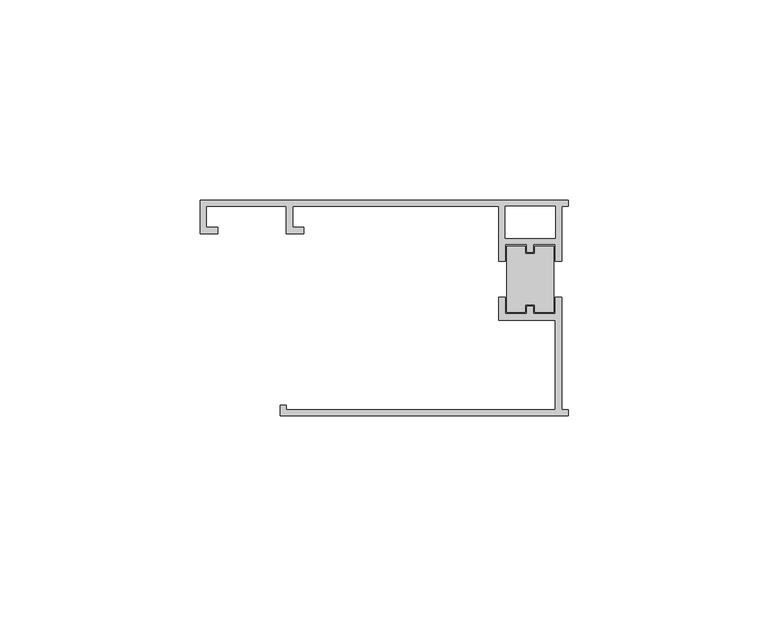
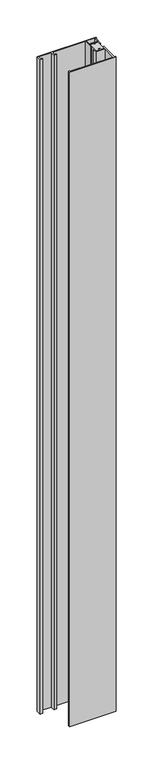
"""IFC4 building model written with IfcOpenShell, lengths in millimetres: proxy geometry, Generic Models 2:Generic Models 2:310765:Generic Models 2:310765 : Generic Models 2:Generic Models 2:310765:59 : Generic Models 2:Generic Models 2:310765:Generic Models 2:310765 : Generic Models 2:Generic Models 2:310765:300385."""

from ifc_helpers import new_model, si_unit, frame, origin, place, context, project, spatial, polyline, outline, extrude, source, transform, mapped, element, save


def generic_models_339765fb(model_context):
    return source(origin(), model_context, "Body", "SweptSolid", [
        extrude(outline(polyline([(564983.3960122, -568246.416762), (564983.3960122, -568229.8645058), (564988.0935108, -568229.8645058), (564988.0935108, -568231.7899212), (564990.4747608, -568231.7899212), (564990.4747608, -568229.8645058), (564995.1722595, -568229.8645058), (564995.1722595, -568246.416762), (564990.4747608, -568246.416762), (564990.4747608, -568244.4913465), (564988.0935108, -568244.4913465), (564988.0935108, -568246.416762), (564983.3960122, -568246.416762)])), frame((0.0, 0.0, 7722.5263373), z_axis=(0.0, 0.0, 1.0), x_axis=(1.0, 0.0, 0.0)), (0.0, 0.0, 1.0), 1078.0747875),
        extrude(outline(polyline([(564906.7441345, -568226.7958673), (564906.7441345, -568218.3494958), (564998.7441345, -568218.3494958), (564998.7441345, -568219.9369958), (564997.1566345, -568219.9369958), (564997.1566345, -568233.6348183), (564995.5691345, -568233.6348183), (564995.5691345, -568229.4676308), (564990.0778858, -568229.4676308), (564990.0778858, -568231.3930462), (564988.4903858, -568231.3930462), (564988.4903858, -568229.4676308), (564982.9991372, -568229.4676308), (564982.9991372, -568233.6348183), (564981.4116372, -568233.6348183), (564981.4116372, -568219.9369958), (564929.9191345, -568219.9369958), (564929.9191345, -568225.2083673), (564932.718961, -568225.2083673), (564932.718961, -568226.7958673), (564928.3316345, -568226.7958673), (564928.3316345, -568219.9369958), (564908.3316345, -568219.9369958), (564908.3316345, -568225.2083673), (564911.131461, -568225.2083673), (564911.131461, -568226.7958673), (564906.7441345, -568226.7958673)]), holes=[polyline([(564982.9991372, -568219.9369958), (564982.9991372, -568227.8801308), (564995.5691345, -568227.8801308), (564995.5691345, -568219.9369958), (564982.9991372, -568219.9369958)])]), frame((0.0, 0.0, 7722.5263373), z_axis=(0.0, 0.0, 1.0), x_axis=(1.0, 0.0, 0.0)), (0.0, 0.0, 1.0), 1078.0747875),
        extrude(outline(polyline([(564998.7441345, -568270.7619958), (564998.7441345, -568272.3494958), (564926.7441345, -568272.3494958), (564926.7441345, -568269.6344059), (564928.3316345, -568269.6344059), (564928.3316345, -568270.7619958), (564995.5691345, -568270.7619958), (564995.5691345, -568248.401137), (564981.4116372, -568248.401137), (564981.4116372, -568242.6464495), (564982.9991372, -568242.6464495), (564982.9991372, -568246.813637), (564988.4903858, -568246.813637), (564988.4903858, -568244.8882215), (564990.0778858, -568244.8882215), (564990.0778858, -568246.813637), (564995.5691345, -568246.813637), (564995.5691345, -568242.6464495), (564997.1566345, -568242.6464495), (564997.1566345, -568270.7619958), (564998.7441345, -568270.7619958)])), frame((0.0, 0.0, 7722.5263373), z_axis=(0.0, 0.0, 1.0), x_axis=(1.0, 0.0, 0.0)), (0.0, 0.0, 1.0), 1078.0747875),
    ])


if __name__ == "__main__":
    model = new_model("IFC4")
    model_context = context("Model", 3, world=origin())
    ifc_project = project(units=[si_unit("LENGTHUNIT", "METRE", prefix="MILLI")], contexts=[model_context])
    site = spatial("IfcSite", under=ifc_project)
    building = spatial("IfcBuilding", under=site)
    placement = place(None, origin())
    generic_models_shape = generic_models_339765fb(model_context)
    element("IfcBuildingElementProxy", 1, Name="Generic Models 2:Generic Models 2:310765:Generic Models 2:310765 : Generic Models 2:Generic Models 2:310765:59 : Generic Models 2:Generic Models 2:310765:Generic Models 2:310765 : Generic Models 2:Generic Models 2:310765:300385", ObjectType="Generic Models 2:Generic Models 2:310765:Generic Models 2:310765 : Generic Models 2:Generic Models 2:310765:59 : Generic Models 2:Generic Models 2:310765:Generic Models 2:310765 : Generic Models 2:Generic Models 2:310765:300385", at=placement, inside=building, context=model_context, shape_type="MappedRepresentation", body=[
        mapped(generic_models_shape, transform((0.0, 0.0, 0.0), x_axis=(1.0, 0.0, 0.0), y_axis=(0.0, 1.0, 0.0), z_axis=(0.0, 0.0, 1.0))),
    ])
    save(model, "model.ifc")

# Revit data of these elements
# Type "Generic Models 2:Generic Models 2:310765:Generic Models 2:310765 : Generic Models 2:Generic Models 2:310765:59 : Generic Models 2:Generic Models 2:310765:Generic Models 2:310765 : Generic Models 2:Generic Models 2:310765:300385"
#   NameOverride = "Generic Models 2:Generic Models 2:310765:Generic Models 2:310765 : Generic Models 2:Generic Models 2:310765:300385"
#   ObjectTypeOverride = "Generic Models 2:310765 : Generic Models 2:Generic Models 2:310765"
#   Reference = "Generic Models 2"
#   Tag = "300385"
# Element 1 (IfcBuildingElementProxy, "Generic Models 2:Generic Models 2:310765:Generic Models 2:310765 : Generic Models 2:Generic Models 2:310765:59 : Generic Models 2:Generic Models 2:310765:Generic Models 2:310765 : Generic Models 2:Generic Models 2:310765:300385")
#   Materials on its faces: "THERMAL BROKEN ALUMINUM STOREFRONT FOR POLYCARBONATE"
# Materials
#   "THERMAL BROKEN ALUMINUM STOREFRONT FOR POLYCARBONATE": class "Unassigned", colour RGB 244 244 244, transparency 0, Keynote = "M07611300.01", Cost = 0
